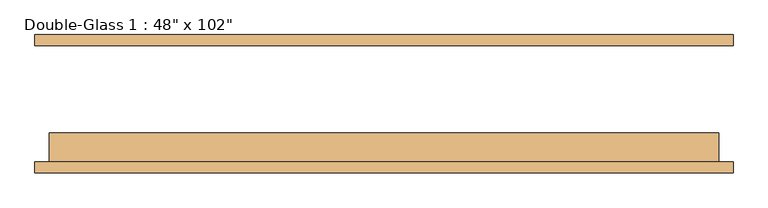
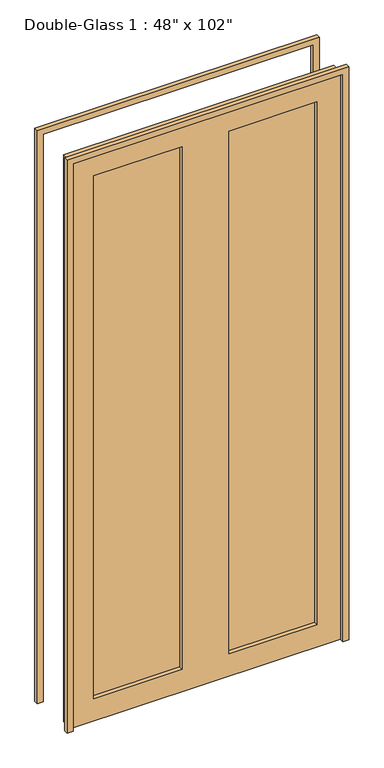
"""IFC4 building model written with IfcOpenShell, lengths in millimetres: door geometry."""

from ifc_helpers import new_model, si_unit, frame, origin, place, context, project, spatial, polyline, outline, extrude, source, transform, mapped, element, save


def door_378294fd(model_context):
    return source(origin(), model_context, "Body", "SweptSolid", [
        extrude(outline(polyline([(0.0, 609.6), (2616.2, 609.6), (2616.2, -609.6), (0.0, -609.6), (0.0, -584.2), (2590.8, -584.2), (2590.8, 584.2), (0.0, 584.2), (0.0, 609.6)])), frame((0.0, 99.21875, 0.0), z_axis=(0.0, 1.0, 0.0), x_axis=(0.0, 0.0, 1.0)), (0.0, 0.0, 1.0), 19.05),
        extrude(outline(polyline([(2590.8, 584.2), (0.0, 584.2), (0.0, 609.6), (2616.2, 609.6), (2616.2, -609.6), (0.0, -609.6), (0.0, -584.2), (2590.8, -584.2), (2590.8, 584.2)])), frame((0.0, -123.03125, 0.0), z_axis=(0.0, 1.0, 0.0), x_axis=(0.0, 0.0, 1.0)), (0.0, 0.0, 1.0), 19.05),
        extrude(outline(polyline([(482.6, -78.58125), (482.6, -85.725), (101.6, -85.725), (101.6, -78.58125), (482.6, -78.58125)])), frame((0.0, 0.0, 101.6), z_axis=(0.0, 0.0, 1.0), x_axis=(1.0, 0.0, 0.0)), (0.0, 0.0, 1.0), 2387.6),
        extrude(outline(polyline([(-101.6, -78.58125), (-101.6, -85.725), (-482.6, -85.725), (-482.6, -78.58125), (-101.6, -78.58125)])), frame((0.0, 0.0, 101.6), z_axis=(0.0, 0.0, 1.0), x_axis=(1.0, 0.0, 0.0)), (0.0, 0.0, 1.0), 2387.6),
        extrude(outline(polyline([(2590.8, 584.2), (2590.8, -584.2), (0.0, -584.2), (0.0, 584.2), (2590.8, 584.2)]), holes=[polyline([(2489.2, -101.6), (101.6, -101.6), (101.6, -482.6), (2489.2, -482.6), (2489.2, -101.6)]), polyline([(2489.2, 482.6), (101.6, 482.6), (101.6, 101.6), (2489.2, 101.6), (2489.2, 482.6)])]), frame((0.0, -103.98125, 0.0), z_axis=(0.0, 1.0, 0.0), x_axis=(0.0, 0.0, 1.0)), (0.0, 0.0, 1.0), 50.8),
    ])


if __name__ == "__main__":
    model = new_model("IFC4")
    model_context = context("Model", 3, world=origin())
    ifc_project = project(units=[si_unit("LENGTHUNIT", "METRE", prefix="MILLI")], contexts=[model_context])
    site = spatial("IfcSite", under=ifc_project)
    building = spatial("IfcBuilding", under=site)
    placement = place(None, origin())
    door_shape = door_378294fd(model_context)
    element("IfcDoor", 1, ObjectType="Double-Glass 1 : 48\" x 102\"", at=placement, inside=building, context=model_context, shape_type="MappedRepresentation", body=[
        mapped(door_shape, transform((0.0, 0.0, 0.0), x_axis=(1.0, 0.0, 0.0), y_axis=(0.0, 1.0, 0.0), z_axis=(0.0, 0.0, 1.0))),
    ])
    save(model, "model.ifc")

# Revit data of these elements
# Type "Double-Glass 1 : 48\" x 102\""
#   Type Mark = "30"
#   Assembly Code = "C1020"
#   Thickness = 0' - 2"
#   Height = 8' - 6"
#   Rail Width - Base = 0' - 4"
#   Rail Width - Top = 0' - 4"
#   Stile Width - Hinge = 0' - 4"
#   Stile Width - Latch = 0' - 4"
#   Trim Projection = 0' - 0 3/4"
#   Trim Width = 0' - 1"
#   Width = 3' - 10"
#   Door Material = Door - Panel
#   Frame Material = Door - Frame
#   Function = (empty or 0)
#   Wall Closure = (empty or 0)
# Element 1 (IfcDoor, "Double-Glass 1 : 48\" x 102\"")
#   Materials on its faces: "Door - Frame", "Door - Panel", "Glass"
# Materials
#   "Door - Panel": class "Wood", colour RGB 210 159 95, transparency 0
#   "Door - Frame": class "Miscellaneous", colour RGB 118 70 51, transparency 0
#   "Glass": class "Glass", colour RGB 0 128 192, transparency 0.75
